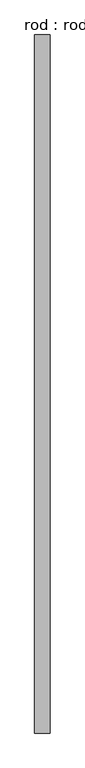
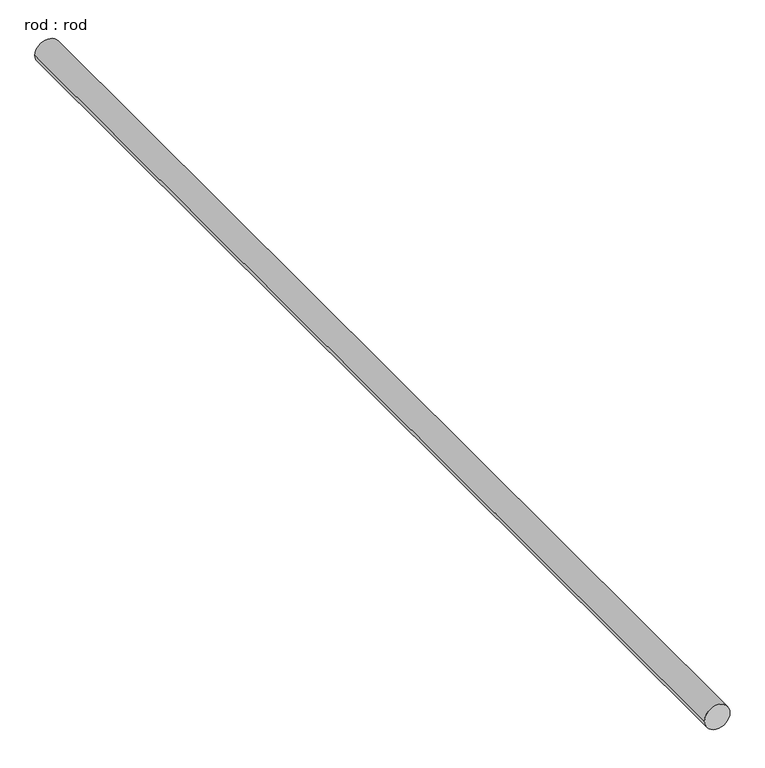
"""IFC4 building model written with IfcOpenShell, lengths in millimetres: proxy geometry, rod : rod."""

from ifc_helpers import new_model, si_unit, point, frame, frame_2d, origin, place, context, project, spatial, circle_curve, trimmed, segment, composite_curve, outline, extrude, source, transform, mapped, element, save


def rod_rod_e89f44aa(model_context):
    return source(origin(), model_context, "Body", "SweptSolid", [
        extrude(outline(composite_curve([segment(trimmed(circle_curve(frame_2d((0.0108462, 0.0)), 200.0), [point((0.0108462, 200.0))], [point((0.0108462, -200.0))], False, "CARTESIAN"), True, "CONTINUOUS"), segment(trimmed(circle_curve(frame_2d((0.0108462, 0.0)), 200.0), [point((0.0108462, -200.0))], [point((0.0108462, 200.0))], False, "CARTESIAN"), True, "CONTINUOUS")], self_intersect=False)), frame((0.0, -5032.2713847, 0.0), z_axis=(0.0, 1.0, 0.0), x_axis=(0.0, 0.0, 1.0)), (0.0, 0.0, 1.0), 18250.0),
    ])


if __name__ == "__main__":
    model = new_model("IFC4")
    model_context = context("Model", 3, world=origin())
    ifc_project = project(units=[si_unit("LENGTHUNIT", "METRE", prefix="MILLI")], contexts=[model_context])
    site = spatial("IfcSite", under=ifc_project)
    building = spatial("IfcBuilding", under=site)
    placement = place(None, origin())
    rod_rod_shape = rod_rod_e89f44aa(model_context)
    element("IfcBuildingElementProxy", 1, Name="rod : rod", ObjectType="rod : rod", at=placement, inside=building, context=model_context, shape_type="MappedRepresentation", body=[
        mapped(rod_rod_shape, transform((0.0, 0.0, 0.0), x_axis=(1.0, 0.0, 0.0), y_axis=(0.0, 1.0, 0.0), z_axis=(0.0, 0.0, 1.0))),
    ])
    save(model, "model.ifc")

# Revit data of these elements
# Type "rod : rod"
#   Default Elevation = 0
